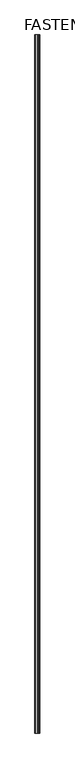
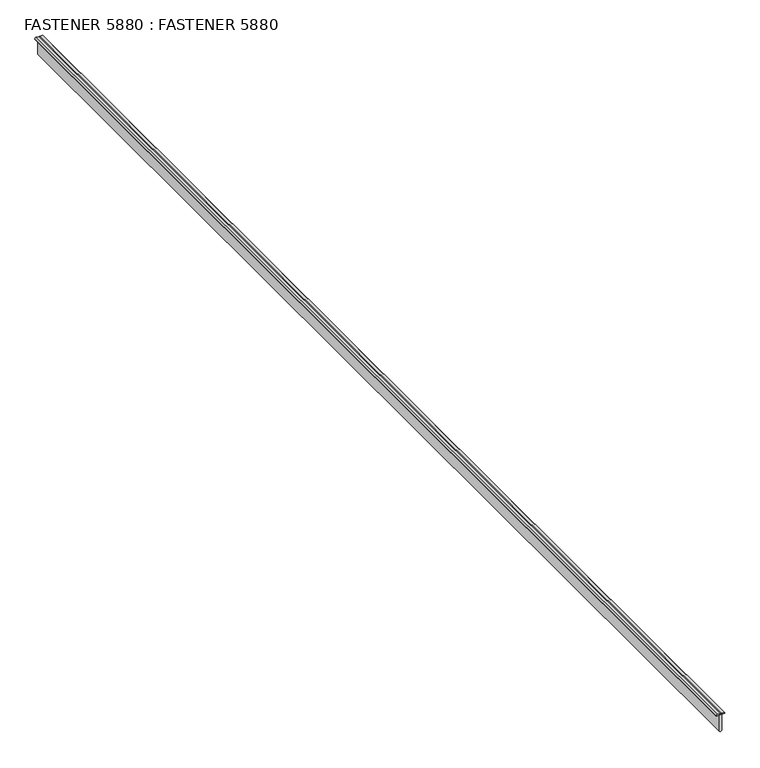
"""IFC4 building model written with IfcOpenShell, lengths in millimetres: proxy geometry, FASTENER 5880 : FASTENER 5880."""

import ifcopenshell
import ifcopenshell.guid

model = None  # the IFC model being written
_history = None  # IfcOwnerHistory: only IFC2X3 demands one
_inside = {}  # id of a spatial element -> (the spatial element, [elements in it])
_under = {}  # id of a project, library or spatial element -> (it, [spatial elements below it])
_declared = {}  # id of a project -> (the project, [libraries it declares])
_typed = {}  # id of a type object -> (the type object, [elements of that type])
_made_of = {}  # id of a material, layer set ... -> (it, [elements and type objects made of it])


def new_model(schema):
    """Start an empty IFC model of exactly this schema.

    Asked for "IFC4X3", IfcOpenShell would pick the latest addendum, in which some entities
    have other attributes; the version numbers below select the first issue.
    IFC2X3 requires an IfcOwnerHistory on every rooted entity: one is made here for all.
    """
    global model, _history
    if schema == "IFC4X3":
        model = ifcopenshell.file(schema_version=(4, 3, 0, 0))
    else:
        model = ifcopenshell.file(schema=schema)
    _inside.clear()
    _under.clear()
    _declared.clear()
    _typed.clear()
    _made_of.clear()
    _history = None
    if model.schema == "IFC2X3":
        org = make("IfcOrganization", Name="unknown")
        user = make(
            "IfcPersonAndOrganization",
            ThePerson=make("IfcPerson", FamilyName="unknown"),
            TheOrganization=org,
        )
        app = make(
            "IfcApplication",
            ApplicationDeveloper=org,
            Version="unknown",
            ApplicationFullName="unknown",
            ApplicationIdentifier="unknown",
        )
        _history = make(
            "IfcOwnerHistory",
            OwningUser=user,
            OwningApplication=app,
            ChangeAction="ADDED",
            CreationDate=0,
        )
    return model


def make(cls, **values):
    """One entity of the class cls with the attributes given. An attribute that is None is left unset."""
    return model.create_entity(
        cls, **{name: value for name, value in values.items() if value is not None}
    )


def rooted(cls, **values):
    """An entity with a GlobalId (a new one), such as an element, a storey or a relation."""
    return make(cls, GlobalId=ifcopenshell.guid.new(), OwnerHistory=_history, **values)


def si_unit(unit_type, name, prefix=None):
    """IfcSIUnit, for example si_unit("LENGTHUNIT", "METRE", prefix="MILLI")."""
    return make("IfcSIUnit", UnitType=unit_type, Prefix=prefix, Name=name)


def assignment(units):
    """IfcUnitAssignment: the units of a project."""
    return None if units is None else make("IfcUnitAssignment", Units=units)


def point(xyz):
    """IfcCartesianPoint."""
    return None if xyz is None else make("IfcCartesianPoint", Coordinates=xyz)


def direction(xyz):
    """IfcDirection."""
    return None if xyz is None else make("IfcDirection", DirectionRatios=xyz)


def frame(location, z_axis=None, x_axis=None):
    """IfcAxis2Placement3D, a coordinate frame: its origin and axes. An axis left out is left unset."""
    return make(
        "IfcAxis2Placement3D",
        Location=point(location),
        Axis=direction(z_axis),
        RefDirection=direction(x_axis),
    )


def origin():
    """The frame at (0, 0, 0) with its axes left unset."""
    return frame((0.0, 0.0, 0.0))


def place(relative_to, where):
    """IfcLocalPlacement: puts the frame where relative to a parent placement (None: the world)."""
    return make(
        "IfcLocalPlacement", PlacementRelTo=relative_to, RelativePlacement=where
    )


def context(
    kind, dimensions, precision=None, world=None, true_north=None, identifier=None
):
    """IfcGeometricRepresentationContext, for example the 3D "Model" context."""
    return make(
        "IfcGeometricRepresentationContext",
        ContextIdentifier=identifier,
        ContextType=kind,
        CoordinateSpaceDimension=dimensions,
        Precision=precision,
        WorldCoordinateSystem=world,
        TrueNorth=true_north,
    )


def project(units=None, contexts=None):
    """IfcProject with its units and contexts."""
    return rooted(
        "IfcProject",
        Name="project",
        RepresentationContexts=contexts,
        UnitsInContext=assignment(units),
    )


def spatial(cls, under=None, at=None, **own):
    """A site, building, storey or space (cls), placed at a placement, below another one or the project."""
    s = rooted(cls, ObjectPlacement=at, **own)
    if under is not None:
        _under.setdefault(under.id(), (under, []))[1].append(s)
    return s


def polyline(points):
    """IfcPolyline through the points."""
    return make("IfcPolyline", Points=[point(p) for p in points])


def outline(outer, holes=None, kind="AREA"):
    """IfcArbitraryClosedProfileDef: a profile drawn as a closed curve; with holes, ...WithVoids."""
    if holes is None:
        return make("IfcArbitraryClosedProfileDef", ProfileType=kind, OuterCurve=outer)
    return make(
        "IfcArbitraryProfileDefWithVoids",
        ProfileType=kind,
        OuterCurve=outer,
        InnerCurves=holes,
    )


def extrude(swept, where, along, depth):
    """IfcExtrudedAreaSolid: the profile swept, set in the frame where, extruded along a direction by depth."""
    return make(
        "IfcExtrudedAreaSolid",
        SweptArea=swept,
        Position=where,
        ExtrudedDirection=direction(along),
        Depth=depth,
    )


def shape(context_of_items, identifier, shape_type, items):
    """IfcShapeRepresentation: the items that make up one representation, for example the "Body"."""
    return make(
        "IfcShapeRepresentation",
        ContextOfItems=context_of_items,
        RepresentationIdentifier=identifier,
        RepresentationType=shape_type,
        Items=items,
    )


def source(mapping_origin, context_of_items, identifier, shape_type, items):
    """IfcRepresentationMap: a shape defined once, which mapped items show again and again."""
    return make(
        "IfcRepresentationMap",
        MappingOrigin=mapping_origin,
        MappedRepresentation=shape(context_of_items, identifier, shape_type, items),
    )


def transform(
    local_origin,
    x_axis=None,
    y_axis=None,
    z_axis=None,
    scale=None,
    scale2=None,
    scale3=None,
    uniform=True,
):
    """IfcCartesianTransformationOperator3D, or its non-uniform kind. x_axis, y_axis, z_axis: its Axis1, 2, 3."""
    if uniform:
        return make(
            "IfcCartesianTransformationOperator3D",
            Axis1=direction(x_axis),
            Axis2=direction(y_axis),
            LocalOrigin=point(local_origin),
            Scale=scale,
            Axis3=direction(z_axis),
        )
    return make(
        "IfcCartesianTransformationOperator3DnonUniform",
        Axis1=direction(x_axis),
        Axis2=direction(y_axis),
        LocalOrigin=point(local_origin),
        Scale=scale,
        Axis3=direction(z_axis),
        Scale2=scale2,
        Scale3=scale3,
    )


def mapped(mapping_source, mapping_target):
    """IfcMappedItem: shows the shape of a source again, moved by a transform."""
    return make(
        "IfcMappedItem", MappingSource=mapping_source, MappingTarget=mapping_target
    )


def made_of(thing, what):
    """Note that an element or type object is made of a material, layer set ...; save() writes the relation."""
    if what is not None:
        _made_of.setdefault(what.id(), (what, []))[1].append(thing)
    return thing


def element(
    cls,
    number,
    at=None,
    inside=None,
    cuts=None,
    type_object=None,
    material=None,
    context=None,
    identifier="Body",
    shape_type=None,
    held_by="IfcProductDefinitionShape",
    body=None,
    shapes=None,
    **own,
):
    """One element of the class cls, such as IfcWall. Its Tag is "e" and its number.

    at: its placement. inside: the storey or other place that contains it. cuts: it is an
    opening in that element (IfcRelVoidsElement). A single representation is given by context,
    identifier, shape_type and body (its items); several are given by shapes. held_by: the class
    of the entity that holds the representations. save() writes the other relations.
    """
    e = rooted(cls, Tag="e%d" % number, ObjectPlacement=at, **own)
    if body is not None:
        shapes = [shape(context, identifier, shape_type, body)]
    if shapes is not None:
        e.Representation = make(held_by, Representations=shapes)
    if inside is not None:
        _inside.setdefault(inside.id(), (inside, []))[1].append(e)
    if cuts is not None:
        rooted(
            "IfcRelVoidsElement", RelatingBuildingElement=cuts, RelatedOpeningElement=e
        )
    if type_object is not None:
        _typed.setdefault(type_object.id(), (type_object, []))[1].append(e)
    return made_of(e, material)


def aggregate(whole, parts):
    """IfcRelAggregates: a whole, such as a stair, and the parts it consists of."""
    return rooted("IfcRelAggregates", RelatingObject=whole, RelatedObjects=parts)


def save(model, path):
    """Write the relations noted so far, then the file.

    IfcRelAggregates (storeys below a building ...), IfcRelContainedInSpatialStructure (elements
    in a storey), IfcRelDefinesByType, IfcRelAssociatesMaterial and IfcRelDeclares: one each for
    every whole, place, type object, material and project.
    """
    for whole, parts in _under.values():
        aggregate(whole, parts)
    for where, things in _inside.values():
        rooted(
            "IfcRelContainedInSpatialStructure",
            RelatedElements=things,
            RelatingStructure=where,
        )
    for kind, things in _typed.values():
        rooted("IfcRelDefinesByType", RelatedObjects=things, RelatingType=kind)
    for what, things in _made_of.values():
        rooted("IfcRelAssociatesMaterial", RelatedObjects=things, RelatingMaterial=what)
    for by, libraries in _declared.values():
        rooted("IfcRelDeclares", RelatingContext=by, RelatedDefinitions=libraries)
    model.write(path)


def fastener_5880_fastener_5880_40db04d7(model_context):
    return source(origin(), model_context, "Body", "SweptSolid", [
        extrude(outline(polyline([(42551.3049701, 5981.517626), (42579.6987049, 5981.517626), (42579.6987049, 5977.3107075), (42550.7399648, 5977.3107075), (42549.1244121, 5978.9677221), (42551.3049701, 5981.517626)])), frame((0.0, -1052.8906574, 0.0), z_axis=(0.0, 1.0, 0.0), x_axis=(0.0, 0.0, 1.0)), (0.0, 0.0, 1.0), 1999.85),
        extrude(outline(polyline([(42580.5349921, 5972.2779845), (42579.6987049, 5972.2671879), (42579.6987049, 5986.5634932), (42580.508527, 5986.5634932), (42582.1023984, 5985.3247911), (42582.1023984, 5980.4457092), (42580.1167322, 5980.0391089), (42580.1167322, 5978.792004), (42581.7222633, 5978.792004), (42582.1288635, 5973.5166866), (42580.5349921, 5972.2779845)])), frame((0.0, -1052.8906574, 0.0), z_axis=(0.0, 1.0, 0.0), x_axis=(0.0, 0.0, 1.0)), (0.0, 0.0, 1.0), 1999.85),
    ])


if __name__ == "__main__":
    model = new_model("IFC4")
    model_context = context("Model", 3, world=origin())
    ifc_project = project(units=[si_unit("LENGTHUNIT", "METRE", prefix="MILLI")], contexts=[model_context])
    site = spatial("IfcSite", under=ifc_project)
    building = spatial("IfcBuilding", under=site)
    placement = place(None, origin())
    fastener_5880_fastener_5880_shape = fastener_5880_fastener_5880_40db04d7(model_context)
    element("IfcBuildingElementProxy", 1, Name="FASTENER 5880 : FASTENER 5880", ObjectType="FASTENER 5880 : FASTENER 5880", at=placement, inside=building, context=model_context, shape_type="MappedRepresentation", body=[
        mapped(fastener_5880_fastener_5880_shape, transform((0.0, 0.0, 0.0), x_axis=(1.0, 0.0, 0.0), y_axis=(0.0, 1.0, 0.0), z_axis=(0.0, 0.0, 1.0))),
    ])
    save(model, "model.ifc")

# Revit data of these elements
# Type "FASTENER 5880 : FASTENER 5880"
#   NameOverride = "FASTENER"
# Element 1 (IfcBuildingElementProxy, "FASTENER 5880 : FASTENER 5880")
#   Materials on its faces: "ENGINEERED PANCAKE HEAD FASTENER (NOT BY AEP-SPAN) @ 12\" O.C."
# Materials
#   "ENGINEERED PANCAKE HEAD FASTENER (NOT BY AEP-SPAN) @ 12\" O.C.": class "Unassigned", colour RGB 255 255 255, transparency 0
